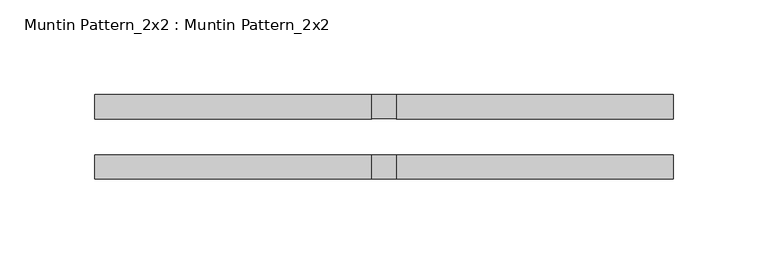
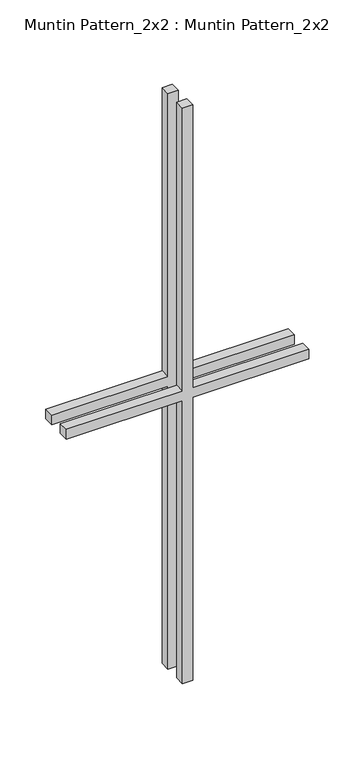
"""IFC4 building model written with IfcOpenShell, lengths in millimetres: proxy geometry, Muntin Pattern_2x2 : Muntin Pattern_2x2."""

from ifc_helpers import new_model, si_unit, frame, origin, place, context, project, spatial, polyline, outline, extrude, source, transform, mapped, element, save


def muntin_pattern_2x2_muntin_pattern_2x2_e055f423(model_context):
    return source(origin(), model_context, "Body", "SweptSolid", [
        extrude(outline(polyline([(388.9375, -6.35), (388.9375, -152.4), (376.2375, -152.4), (376.2375, -6.35), (0.0, -6.35), (0.0, 6.35), (376.2375, 6.35), (376.2375, 152.4), (388.9375, 152.4), (388.9375, 6.35), (765.175, 6.35), (765.175, -6.35), (388.9375, -6.35)])), frame((0.0, 9.525, 0.0), z_axis=(0.0, 1.0, 0.0), x_axis=(0.0, 0.0, 1.0)), (0.0, 0.0, 1.0), 12.7),
        extrude(outline(polyline([(388.9375, -6.35), (388.9375, -152.4), (376.2375, -152.4), (376.2375, -6.35), (0.0, -6.35), (0.0, 6.35), (376.2375, 6.35), (376.2375, 152.4), (388.9375, 152.4), (388.9375, 6.35), (765.175, 6.35), (765.175, -6.35), (388.9375, -6.35)])), frame((0.0, -22.225, 0.0), z_axis=(0.0, 1.0, 0.0), x_axis=(0.0, 0.0, 1.0)), (0.0, 0.0, 1.0), 12.7),
    ])


if __name__ == "__main__":
    model = new_model("IFC4")
    model_context = context("Model", 3, world=origin())
    ifc_project = project(units=[si_unit("LENGTHUNIT", "METRE", prefix="MILLI")], contexts=[model_context])
    site = spatial("IfcSite", under=ifc_project)
    building = spatial("IfcBuilding", under=site)
    placement = place(None, origin())
    muntin_pattern_2x2_muntin_pattern_2x2_shape = muntin_pattern_2x2_muntin_pattern_2x2_e055f423(model_context)
    element("IfcBuildingElementProxy", 1, Name="Muntin Pattern_2x2 : Muntin Pattern_2x2", ObjectType="Muntin Pattern_2x2 : Muntin Pattern_2x2", at=placement, inside=building, context=model_context, shape_type="MappedRepresentation", body=[
        mapped(muntin_pattern_2x2_muntin_pattern_2x2_shape, transform((0.0, 0.0, 0.0), x_axis=(1.0, 0.0, 0.0), y_axis=(0.0, 1.0, 0.0), z_axis=(0.0, 0.0, 1.0))),
    ])
    save(model, "model.ifc")

# Revit data of these elements
# Type "Muntin Pattern_2x2 : Muntin Pattern_2x2"
#   Width [instance default] = 4' - 0"
#   Thickness = 0' - 0 1/2"
#   Height [instance default] = 4' - 0"
#   Distance = 0' - 0 3/4"
#   Interior Material [instance default] = none
#   Exterior Material [instance default] = none
# Element 1 (IfcBuildingElementProxy, "Muntin Pattern_2x2 : Muntin Pattern_2x2")
#   Width = 1' - 0"
#   Height = 2' - 6 1/8"
#   Interior Material = Wood - Stained
#   Exterior Material = Clad - White
#   Materials on its faces: "Clad - White", "Wood - Stained"
# Materials
#   "Clad - White": class "Wood", colour RGB 242 242 238, transparency 0, Cost = 0
#   "Wood - Stained": class "Wood", colour RGB 224 178 126, transparency 0, Cost = 0
